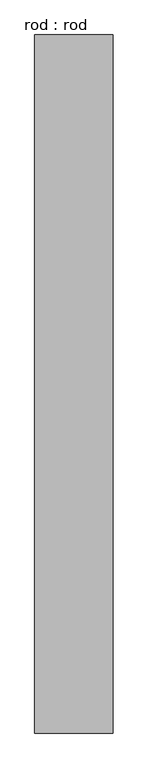
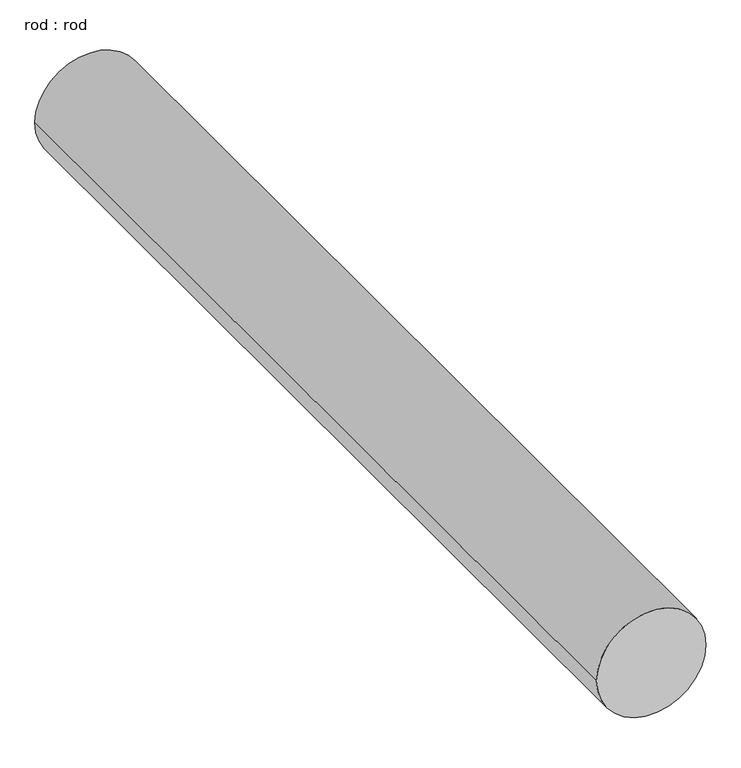
"""IFC4 building model written with IfcOpenShell, lengths in millimetres: proxy geometry, rod : rod."""

from ifc_helpers import new_model, si_unit, point, frame, frame_2d, origin, place, context, project, spatial, circle_curve, trimmed, segment, composite_curve, outline, extrude, source, transform, mapped, element, save


def rod_rod_d6486d7b(model_context):
    return source(origin(), model_context, "Body", "SweptSolid", [
        extrude(outline(composite_curve([segment(trimmed(circle_curve(frame_2d((0.0108462, 0.0)), 200.0), [point((0.0108462, 200.0))], [point((0.0108462, -200.0))], False, "CARTESIAN"), True, "CONTINUOUS"), segment(trimmed(circle_curve(frame_2d((0.0108462, 0.0)), 200.0), [point((0.0108462, -200.0))], [point((0.0108462, 200.0))], False, "CARTESIAN"), True, "CONTINUOUS")], self_intersect=False)), frame((0.0, 2314.1571868, 0.0), z_axis=(0.0, 1.0, 0.0), x_axis=(0.0, 0.0, 1.0)), (0.0, 0.0, 1.0), 3557.1428571),
    ])


if __name__ == "__main__":
    model = new_model("IFC4")
    model_context = context("Model", 3, world=origin())
    ifc_project = project(units=[si_unit("LENGTHUNIT", "METRE", prefix="MILLI")], contexts=[model_context])
    site = spatial("IfcSite", under=ifc_project)
    building = spatial("IfcBuilding", under=site)
    placement = place(None, origin())
    rod_rod_shape = rod_rod_d6486d7b(model_context)
    element("IfcBuildingElementProxy", 1, Name="rod : rod", ObjectType="rod : rod", at=placement, inside=building, context=model_context, shape_type="MappedRepresentation", body=[
        mapped(rod_rod_shape, transform((0.0, 0.0, 0.0), x_axis=(1.0, 0.0, 0.0), y_axis=(0.0, 1.0, 0.0), z_axis=(0.0, 0.0, 1.0))),
    ])
    save(model, "model.ifc")

# Revit data of these elements
# Type "rod : rod"
#   Default Elevation = 0
